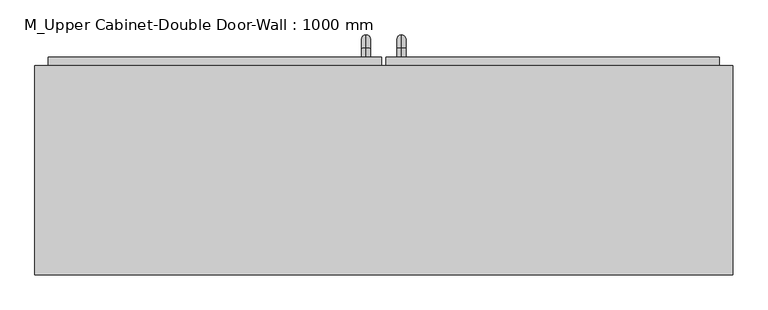
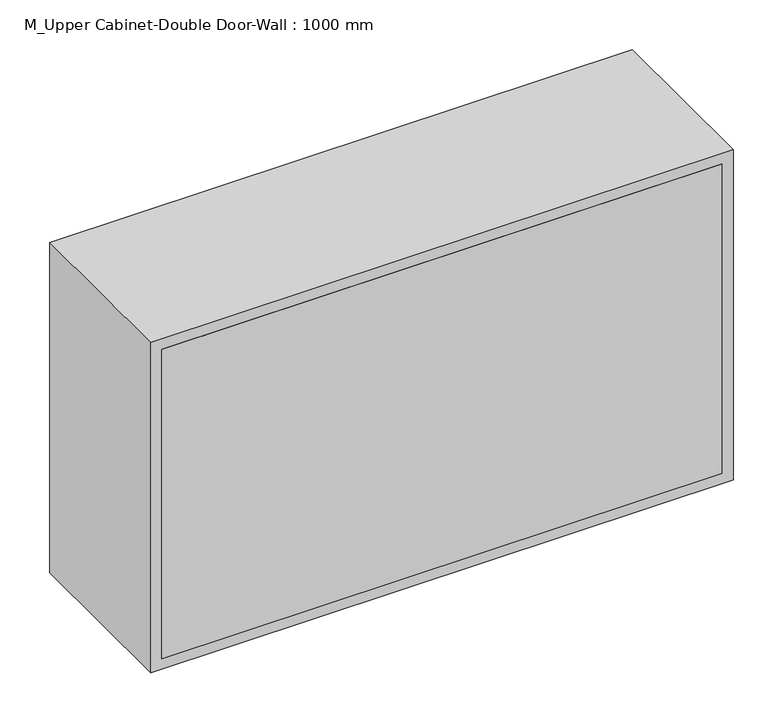
"""IFC4 building model written with IfcOpenShell, lengths in millimetres: furniture geometry, M_Upper Cabinet-Double Door-Wall : 1000 mm."""

from ifc_helpers import new_model, si_unit, point, frame, origin, place, context, project, spatial, polyline, circle_curve, ellipse_curve, trimmed, outline, extrude, source, transform, mapped, element, save
from ifc_brep_helpers import plane_surface, cylinder_surface, revolved_surface, advanced_brep


def m_upper_cabinet_double_door_wall_1000_mm_b8e39643(model_context):
    return source(origin(), model_context, "Body", "SolidModel", [
        advanced_brep(
        [(55.1711628, 388.7, 1546.05), (55.1711628, 388.7, 1558.75), (55.1711628, 401.4, 1546.05), (55.1711628, 401.4, 1558.75), (55.1711628, 420.45, 1539.7), (55.1711628, 407.75, 1539.7), (55.1711628, 407.75, 1463.5), (55.1711628, 420.45, 1463.5), (55.1711628, 401.4, 1444.45), (55.1711628, 401.4, 1457.15), (55.1711628, 388.7, 1457.15), (55.1711628, 388.7, 1444.45)],
        [
            (0, 1, circle_curve(frame((55.1711628, 388.7, 1552.4), z_axis=(0.0, -1.0, 0.0), x_axis=(0.0, 0.0, -1.0)), 6.35)),
            (1, 0, circle_curve(frame((55.1711628, 388.7, 1552.4), z_axis=(0.0, -1.0, 0.0), x_axis=(0.0, 0.0, -1.0)), 6.35)),
            (0, 2),
            (2, 3, circle_curve(frame((55.1711628, 401.4, 1552.4), z_axis=(0.0, -1.0, 0.0), x_axis=(0.0, 0.0, -1.0)), 6.35)),
            (3, 1),
            (3, 2, circle_curve(frame((55.1711628, 401.4, 1552.4), z_axis=(0.0, -1.0, 0.0), x_axis=(0.0, 0.0, -1.0)), 6.35)),
            (4, 3, circle_curve(frame((55.1711628, 401.4, 1539.7), z_axis=(1.0, 0.0, 0.0), x_axis=(0.0, 0.0, 1.0)), 19.05)),
            (2, 5, circle_curve(frame((55.1711628, 401.4, 1539.7), z_axis=(-1.0, 0.0, 0.0), x_axis=(0.0, 0.0, 1.0)), 6.35)),
            (5, 4, circle_curve(frame((55.1711628, 414.1, 1539.7), z_axis=(0.0, 0.0, 1.0), x_axis=(0.0, -1.0, 0.0)), 6.35)),
            (4, 5, circle_curve(frame((55.1711628, 414.1, 1539.7), z_axis=(0.0, 0.0, 1.0), x_axis=(0.0, -1.0, 0.0)), 6.35)),
            (5, 6),
            (6, 7, circle_curve(frame((55.1711628, 414.1, 1463.5), z_axis=(0.0, 0.0, 1.0), x_axis=(0.0, -1.0, 0.0)), 6.35)),
            (7, 4),
            (7, 6, circle_curve(frame((55.1711628, 414.1, 1463.5), z_axis=(0.0, 0.0, 1.0), x_axis=(0.0, -1.0, 0.0)), 6.35)),
            (8, 7, circle_curve(frame((55.1711628, 401.4, 1463.5), z_axis=(1.0, 0.0, 0.0), x_axis=(0.0, 1.0, 0.0)), 19.05)),
            (6, 9, circle_curve(frame((55.1711628, 401.4, 1463.5), z_axis=(-1.0, 0.0, 0.0), x_axis=(0.0, 1.0, 0.0)), 6.35)),
            (9, 8, circle_curve(frame((55.1711628, 401.4, 1450.8), z_axis=(0.0, 1.0, 0.0), x_axis=(0.0, 0.0, 1.0)), 6.35)),
            (8, 9, circle_curve(frame((55.1711628, 401.4, 1450.8), z_axis=(0.0, 1.0, 0.0), x_axis=(0.0, 0.0, 1.0)), 6.35)),
            (10, 11, circle_curve(frame((55.1711628, 388.7, 1450.8), z_axis=(0.0, -1.0, 0.0), x_axis=(0.0, 0.0, 1.0)), 6.35)),
            (11, 10, circle_curve(frame((55.1711628, 388.7, 1450.8), z_axis=(0.0, -1.0, 0.0), x_axis=(0.0, 0.0, 1.0)), 6.35)),
            (9, 10),
            (11, 8),
        ],
        [
            plane_surface(frame((48.8211628, 388.7, 1552.4), z_axis=(0.0, -1.0, 0.0), x_axis=(0.0, 0.0, 1.0))),
            cylinder_surface(frame((55.1711628, 388.7, 1552.4), z_axis=(0.0, -1.0, 0.0), x_axis=(0.0, 0.0, -1.0)), 6.35),
            revolved_surface(trimmed(ellipse_curve(frame((55.1711628, 401.4, 1552.4), z_axis=(0.0, -1.0, 0.0), x_axis=(0.0, 0.0, -1.0)), 6.35, 6.35), [point((55.1711628, 401.4, 1546.05))], [point((55.1711628, 401.4, 1558.75))], True, "CARTESIAN"), (55.1711628, 401.4, 1539.7), (-1.0, 0.0, 0.0)),
            revolved_surface(trimmed(ellipse_curve(frame((55.1711628, 401.4, 1552.4), z_axis=(0.0, -1.0, 0.0), x_axis=(0.0, 0.0, -1.0)), 6.35, 6.35), [point((55.1711628, 401.4, 1558.75))], [point((55.1711628, 401.4, 1546.05))], True, "CARTESIAN"), (55.1711628, 401.4, 1539.7), (-1.0, 0.0, 0.0)),
            cylinder_surface(frame((55.1711628, 414.1, 1539.7), z_axis=(0.0, 0.0, 1.0), x_axis=(0.0, -1.0, 0.0)), 6.35),
            revolved_surface(trimmed(ellipse_curve(frame((55.1711628, 414.1, 1463.5), z_axis=(0.0, 0.0, 1.0), x_axis=(0.0, -1.0, 0.0)), 6.35, 6.35), [point((55.1711628, 407.75, 1463.5))], [point((55.1711628, 420.45, 1463.5))], True, "CARTESIAN"), (55.1711628, 401.4, 1463.5), (-1.0, 0.0, 0.0)),
            revolved_surface(trimmed(ellipse_curve(frame((55.1711628, 414.1, 1463.5), z_axis=(0.0, 0.0, 1.0), x_axis=(0.0, -1.0, 0.0)), 6.35, 6.35), [point((55.1711628, 420.45, 1463.5))], [point((55.1711628, 407.75, 1463.5))], True, "CARTESIAN"), (55.1711628, 401.4, 1463.5), (-1.0, 0.0, 0.0)),
            plane_surface(frame((48.8211628, 388.7, 1450.8), z_axis=(0.0, -1.0, 0.0), x_axis=(0.0, 0.0, -1.0))),
            cylinder_surface(frame((55.1711628, 401.4, 1450.8), z_axis=(0.0, 1.0, 0.0), x_axis=(0.0, 0.0, 1.0)), 6.35),
        ],
        [
            (0, [[1, 2]]),
            (1, [[-1, 3, 4, 5]]),
            (1, [[-2, -5, 6, -3]]),
            (2, [[7, -4, 8, 9]]),
            (3, [[-8, -6, -7, 10]]),
            (4, [[-9, 11, 12, 13]]),
            (4, [[-10, -13, 14, -11]]),
            (5, [[15, -12, 16, 17]]),
            (6, [[-16, -14, -15, 18]]),
            (7, [[19, 20]]),
            (8, [[-17, 21, -20, 22]]),
            (8, [[-18, -22, -19, -21]]),
        ],
    ),
        advanced_brep(
        [(4.3711628, 388.7, 1546.05), (4.3711628, 388.7, 1558.75), (4.3711628, 401.4, 1546.05), (4.3711628, 401.4, 1558.75), (4.3711628, 420.45, 1539.7), (4.3711628, 407.75, 1539.7), (4.3711628, 407.75, 1463.5), (4.3711628, 420.45, 1463.5), (4.3711628, 401.4, 1444.45), (4.3711628, 401.4, 1457.15), (4.3711628, 388.7, 1457.15), (4.3711628, 388.7, 1444.45)],
        [
            (0, 1, circle_curve(frame((4.3711628, 388.7, 1552.4), z_axis=(0.0, -1.0, 0.0), x_axis=(0.0, 0.0, 1.0)), 6.35)),
            (1, 0, circle_curve(frame((4.3711628, 388.7, 1552.4), z_axis=(0.0, -1.0, 0.0), x_axis=(0.0, 0.0, 1.0)), 6.35)),
            (0, 2),
            (2, 3, circle_curve(frame((4.3711628, 401.4, 1552.4), z_axis=(0.0, -1.0, 0.0), x_axis=(0.0, 0.0, 1.0)), 6.35)),
            (3, 1),
            (3, 2, circle_curve(frame((4.3711628, 401.4, 1552.4), z_axis=(0.0, -1.0, 0.0), x_axis=(0.0, 0.0, 1.0)), 6.35)),
            (4, 3, circle_curve(frame((4.3711628, 401.4, 1539.7), z_axis=(1.0, 0.0, 0.0), x_axis=(0.0, 0.0, 1.0)), 19.05)),
            (2, 5, circle_curve(frame((4.3711628, 401.4, 1539.7), z_axis=(-1.0, 0.0, 0.0), x_axis=(0.0, 0.0, 1.0)), 6.35)),
            (5, 4, circle_curve(frame((4.3711628, 414.1, 1539.7), z_axis=(0.0, 0.0, 1.0), x_axis=(0.0, 1.0, 0.0)), 6.35)),
            (4, 5, circle_curve(frame((4.3711628, 414.1, 1539.7), z_axis=(0.0, 0.0, 1.0), x_axis=(0.0, 1.0, 0.0)), 6.35)),
            (5, 6),
            (6, 7, circle_curve(frame((4.3711628, 414.1, 1463.5), z_axis=(0.0, 0.0, 1.0), x_axis=(0.0, 1.0, 0.0)), 6.35)),
            (7, 4),
            (7, 6, circle_curve(frame((4.3711628, 414.1, 1463.5), z_axis=(0.0, 0.0, 1.0), x_axis=(0.0, 1.0, 0.0)), 6.35)),
            (8, 7, circle_curve(frame((4.3711628, 401.4, 1463.5), z_axis=(1.0, 0.0, 0.0), x_axis=(0.0, 1.0, 0.0)), 19.05)),
            (6, 9, circle_curve(frame((4.3711628, 401.4, 1463.5), z_axis=(-1.0, 0.0, 0.0), x_axis=(0.0, 1.0, 0.0)), 6.35)),
            (9, 8, circle_curve(frame((4.3711628, 401.4, 1450.8), z_axis=(0.0, 1.0, 0.0), x_axis=(0.0, 0.0, -1.0)), 6.35)),
            (8, 9, circle_curve(frame((4.3711628, 401.4, 1450.8), z_axis=(0.0, 1.0, 0.0), x_axis=(0.0, 0.0, -1.0)), 6.35)),
            (10, 11, circle_curve(frame((4.3711628, 388.7, 1450.8), z_axis=(0.0, -1.0, 0.0), x_axis=(0.0, 0.0, -1.0)), 6.35)),
            (11, 10, circle_curve(frame((4.3711628, 388.7, 1450.8), z_axis=(0.0, -1.0, 0.0), x_axis=(0.0, 0.0, -1.0)), 6.35)),
            (9, 10),
            (11, 8),
        ],
        [
            plane_surface(frame((-1.9788372, 388.7, 1552.4), z_axis=(0.0, -1.0, 0.0), x_axis=(0.0, 0.0, 1.0))),
            cylinder_surface(frame((4.3711628, 388.7, 1552.4), z_axis=(0.0, -1.0, 0.0), x_axis=(0.0, 0.0, 1.0)), 6.35),
            revolved_surface(trimmed(ellipse_curve(frame((4.3711628, 401.4, 1552.4), z_axis=(0.0, -1.0, 0.0), x_axis=(0.0, 0.0, 1.0)), 6.35, 6.35), [point((4.3711628, 401.4, 1546.05))], [point((4.3711628, 401.4, 1558.75))], True, "CARTESIAN"), (4.3711628, 401.4, 1539.7), (-1.0, 0.0, 0.0)),
            revolved_surface(trimmed(ellipse_curve(frame((4.3711628, 401.4, 1552.4), z_axis=(0.0, -1.0, 0.0), x_axis=(0.0, 0.0, 1.0)), 6.35, 6.35), [point((4.3711628, 401.4, 1558.75))], [point((4.3711628, 401.4, 1546.05))], True, "CARTESIAN"), (4.3711628, 401.4, 1539.7), (-1.0, 0.0, 0.0)),
            cylinder_surface(frame((4.3711628, 414.1, 1539.7), z_axis=(0.0, 0.0, 1.0), x_axis=(0.0, 1.0, 0.0)), 6.35),
            revolved_surface(trimmed(ellipse_curve(frame((4.3711628, 414.1, 1463.5), z_axis=(0.0, 0.0, 1.0), x_axis=(0.0, 1.0, 0.0)), 6.35, 6.35), [point((4.3711628, 407.75, 1463.5))], [point((4.3711628, 420.45, 1463.5))], True, "CARTESIAN"), (4.3711628, 401.4, 1463.5), (-1.0, 0.0, 0.0)),
            revolved_surface(trimmed(ellipse_curve(frame((4.3711628, 414.1, 1463.5), z_axis=(0.0, 0.0, 1.0), x_axis=(0.0, 1.0, 0.0)), 6.35, 6.35), [point((4.3711628, 420.45, 1463.5))], [point((4.3711628, 407.75, 1463.5))], True, "CARTESIAN"), (4.3711628, 401.4, 1463.5), (-1.0, 0.0, 0.0)),
            plane_surface(frame((-1.9788372, 388.7, 1450.8), z_axis=(0.0, -1.0, 0.0), x_axis=(0.0, 0.0, -1.0))),
            cylinder_surface(frame((4.3711628, 401.4, 1450.8), z_axis=(0.0, 1.0, 0.0), x_axis=(0.0, 0.0, -1.0)), 6.35),
        ],
        [
            (0, [[1, 2]]),
            (1, [[-1, 3, 4, 5]]),
            (1, [[-2, -5, 6, -3]]),
            (2, [[7, -4, 8, 9]]),
            (3, [[-8, -6, -7, 10]]),
            (4, [[-9, 11, 12, 13]]),
            (4, [[-10, -13, 14, -11]]),
            (5, [[15, -12, 16, 17]]),
            (6, [[-16, -14, -15, 18]]),
            (7, [[19, 20]]),
            (8, [[-17, 21, -20, 22]]),
            (8, [[-18, -22, -19, -21]]),
        ],
    ),
        extrude(outline(polyline([(32.9461628, 388.7), (510.7211628, 388.7), (510.7211628, 356.95), (32.9461628, 356.95), (32.9461628, 388.7)])), frame((0.0, 0.0, 1419.05), z_axis=(0.0, 0.0, 1.0), x_axis=(1.0, 0.0, 0.0)), (0.0, 0.0, 1.0), 561.9),
        extrude(outline(polyline([(-451.1788372, 388.7), (26.5961628, 388.7), (26.5961628, 356.95), (-451.1788372, 356.95), (-451.1788372, 388.7)])), frame((0.0, 0.0, 1419.05), z_axis=(0.0, 0.0, 1.0), x_axis=(1.0, 0.0, 0.0)), (0.0, 0.0, 1.0), 561.9),
        extrude(outline(polyline([(510.7211628, 76.0), (-451.1788372, 76.0), (-451.1788372, 95.05), (510.7211628, 95.05), (510.7211628, 76.0)])), frame((0.0, 0.0, 1419.05), z_axis=(0.0, 0.0, 1.0), x_axis=(1.0, 0.0, 0.0)), (0.0, 0.0, 1.0), 561.9),
        extrude(outline(polyline([(2000.0, -470.2288372), (1400.0, -470.2288372), (1400.0, 529.7711628), (2000.0, 529.7711628), (2000.0, -470.2288372)]), holes=[polyline([(1980.95, -451.1788372), (1980.95, 510.7211628), (1419.05, 510.7211628), (1419.05, -451.1788372), (1980.95, -451.1788372)])]), frame((0.0, 76.0, 0.0), z_axis=(0.0, 1.0, 0.0), x_axis=(0.0, 0.0, 1.0)), (0.0, 0.0, 1.0), 300.0),
    ])


if __name__ == "__main__":
    model = new_model("IFC4")
    model_context = context("Model", 3, world=origin())
    ifc_project = project(units=[si_unit("LENGTHUNIT", "METRE", prefix="MILLI")], contexts=[model_context])
    site = spatial("IfcSite", under=ifc_project)
    building = spatial("IfcBuilding", under=site)
    placement = place(None, origin())
    m_upper_cabinet_double_door_wall_1000_mm_shape = m_upper_cabinet_double_door_wall_1000_mm_b8e39643(model_context)
    element("IfcFurniture", 1, ObjectType="M_Upper Cabinet-Double Door-Wall : 1000 mm", at=placement, inside=building, context=model_context, shape_type="MappedRepresentation", body=[
        mapped(m_upper_cabinet_double_door_wall_1000_mm_shape, transform((0.0, 0.0, 0.0), x_axis=(1.0, 0.0, 0.0), y_axis=(0.0, 1.0, 0.0), z_axis=(0.0, 0.0, 1.0))),
    ])
    save(model, "model.ifc")

# Revit data of these elements
# Type "M_Upper Cabinet-Double Door-Wall : 1000 mm"
#   Manufacturer = "Manufacturer"
#   Finish = "Finish"
#   Construction Type = "Construction Type"
#   AccessibilityPerformance = "AccessibilityPerformance"
#   CodePerformance = "CodePerformance"
#   Area = "Area"
#   Color = "Color"
#   Constituents = "Constituents"
#   Features = "Features"
#   Finish = "Finish"
#   Grade = "Grade"
#   Material = "Material"
#   ModelReference = "ModelReference"
#   NominalHeight = "NominalHeight"
#   NominalLength = "NominalLength"
#   NominalWidth = "NominalWidth"
#   ProductionYear = "ProductionYear"
#   Reference = "Reference"
#   Shape = "Shape"
#   Size = "Size"
#   SustainabilityPerformance = "SustainabilityPerformance"
#   WarrantyDescription = "WarrantyDescription"
#   WarrantyDurationLabor = "WarrantyDurationLabor"
#   WarrantyDurationParts = "WarrantyDurationParts"
#   WarrantyGuarantorLabor = "WarrantyGuarantorLabor"
#   WarrantyGuarantorParts = "WarrantyGuarantorParts"
#   ExpectedLife = "ExpectedLife"
#   ReplacementCost = "ReplacementCost"
#   AssetAccountingType = "FIXED"
#   ModelLabel = "ModelLabel"
#   Depth = 0.300 m
#   Height = 0.600 m
#   Top Of Cabinet = 2.000 m
#   Width = 1.000 m
#   Cabinet Material = none
#   Door/Drawer Material = none
#   Handle Material = Cabinets - Handles
# Element 1 (IfcFurniture, "M_Upper Cabinet-Double Door-Wall : 1000 mm")
#   Materials on its faces: "Cabinets", "Cabinets - Handles"
# Materials
#   "Cabinets - Handles": class "Metal", colour RGB 57 57 57, transparency 0
#   "Cabinets": class "Miscellaneous", colour RGB 249 249 249, transparency 0
